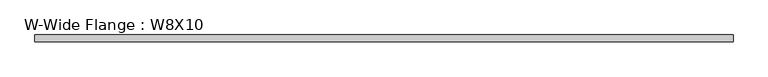
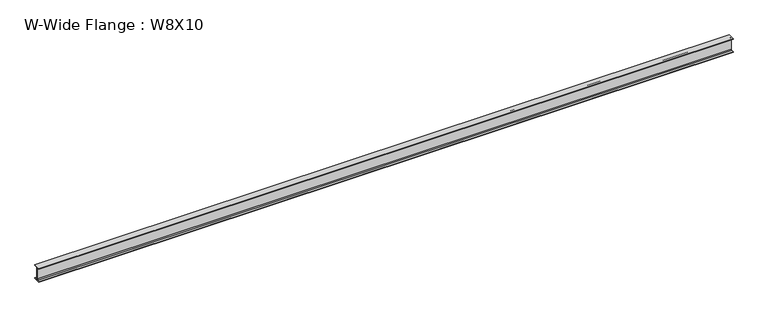
"""IFC4 building model written with IfcOpenShell, lengths in millimetres: beam geometry, W-Wide Flange : W8X10."""

import ifcopenshell
import ifcopenshell.guid

model = None  # the IFC model being written
_history = None  # IfcOwnerHistory: only IFC2X3 demands one
_inside = {}  # id of a spatial element -> (the spatial element, [elements in it])
_under = {}  # id of a project, library or spatial element -> (it, [spatial elements below it])
_declared = {}  # id of a project -> (the project, [libraries it declares])
_typed = {}  # id of a type object -> (the type object, [elements of that type])
_made_of = {}  # id of a material, layer set ... -> (it, [elements and type objects made of it])


def new_model(schema):
    """Start an empty IFC model of exactly this schema.

    Asked for "IFC4X3", IfcOpenShell would pick the latest addendum, in which some entities
    have other attributes; the version numbers below select the first issue.
    IFC2X3 requires an IfcOwnerHistory on every rooted entity: one is made here for all.
    """
    global model, _history
    if schema == "IFC4X3":
        model = ifcopenshell.file(schema_version=(4, 3, 0, 0))
    else:
        model = ifcopenshell.file(schema=schema)
    _inside.clear()
    _under.clear()
    _declared.clear()
    _typed.clear()
    _made_of.clear()
    _history = None
    if model.schema == "IFC2X3":
        org = make("IfcOrganization", Name="unknown")
        user = make(
            "IfcPersonAndOrganization",
            ThePerson=make("IfcPerson", FamilyName="unknown"),
            TheOrganization=org,
        )
        app = make(
            "IfcApplication",
            ApplicationDeveloper=org,
            Version="unknown",
            ApplicationFullName="unknown",
            ApplicationIdentifier="unknown",
        )
        _history = make(
            "IfcOwnerHistory",
            OwningUser=user,
            OwningApplication=app,
            ChangeAction="ADDED",
            CreationDate=0,
        )
    return model


def make(cls, **values):
    """One entity of the class cls with the attributes given. An attribute that is None is left unset."""
    return model.create_entity(
        cls, **{name: value for name, value in values.items() if value is not None}
    )


def rooted(cls, **values):
    """An entity with a GlobalId (a new one), such as an element, a storey or a relation."""
    return make(cls, GlobalId=ifcopenshell.guid.new(), OwnerHistory=_history, **values)


def si_unit(unit_type, name, prefix=None):
    """IfcSIUnit, for example si_unit("LENGTHUNIT", "METRE", prefix="MILLI")."""
    return make("IfcSIUnit", UnitType=unit_type, Prefix=prefix, Name=name)


def assignment(units):
    """IfcUnitAssignment: the units of a project."""
    return None if units is None else make("IfcUnitAssignment", Units=units)


def point(xyz):
    """IfcCartesianPoint."""
    return None if xyz is None else make("IfcCartesianPoint", Coordinates=xyz)


def direction(xyz):
    """IfcDirection."""
    return None if xyz is None else make("IfcDirection", DirectionRatios=xyz)


def frame(location, z_axis=None, x_axis=None):
    """IfcAxis2Placement3D, a coordinate frame: its origin and axes. An axis left out is left unset."""
    return make(
        "IfcAxis2Placement3D",
        Location=point(location),
        Axis=direction(z_axis),
        RefDirection=direction(x_axis),
    )


def frame_2d(location, x_axis=None):
    """IfcAxis2Placement2D, a coordinate frame in the plane: its origin and x axis."""
    return make(
        "IfcAxis2Placement2D", Location=point(location), RefDirection=direction(x_axis)
    )


def origin():
    """The frame at (0, 0, 0) with its axes left unset."""
    return frame((0.0, 0.0, 0.0))


def place(relative_to, where):
    """IfcLocalPlacement: puts the frame where relative to a parent placement (None: the world)."""
    return make(
        "IfcLocalPlacement", PlacementRelTo=relative_to, RelativePlacement=where
    )


def context(
    kind, dimensions, precision=None, world=None, true_north=None, identifier=None
):
    """IfcGeometricRepresentationContext, for example the 3D "Model" context."""
    return make(
        "IfcGeometricRepresentationContext",
        ContextIdentifier=identifier,
        ContextType=kind,
        CoordinateSpaceDimension=dimensions,
        Precision=precision,
        WorldCoordinateSystem=world,
        TrueNorth=true_north,
    )


def project(units=None, contexts=None):
    """IfcProject with its units and contexts."""
    return rooted(
        "IfcProject",
        Name="project",
        RepresentationContexts=contexts,
        UnitsInContext=assignment(units),
    )


def spatial(cls, under=None, at=None, **own):
    """A site, building, storey or space (cls), placed at a placement, below another one or the project."""
    s = rooted(cls, ObjectPlacement=at, **own)
    if under is not None:
        _under.setdefault(under.id(), (under, []))[1].append(s)
    return s


def polyline(points):
    """IfcPolyline through the points."""
    return make("IfcPolyline", Points=[point(p) for p in points])


def circle_curve(where, radius):
    """IfcCircle in the frame where."""
    return make("IfcCircle", Position=where, Radius=radius)


def trimmed(basis, trim1, trim2, sense, master):
    """IfcTrimmedCurve: the piece of a basis curve between two trims."""
    return make(
        "IfcTrimmedCurve",
        BasisCurve=basis,
        Trim1=trim1,
        Trim2=trim2,
        SenseAgreement=sense,
        MasterRepresentation=master,
    )


def segment(curve, same_sense, transition):
    """IfcCompositeCurveSegment."""
    return make(
        "IfcCompositeCurveSegment",
        Transition=transition,
        SameSense=same_sense,
        ParentCurve=curve,
    )


def composite_curve(segments, self_intersect=None):
    """IfcCompositeCurve: segments joined end to end."""
    return make("IfcCompositeCurve", Segments=segments, SelfIntersect=self_intersect)


def outline(outer, holes=None, kind="AREA"):
    """IfcArbitraryClosedProfileDef: a profile drawn as a closed curve; with holes, ...WithVoids."""
    if holes is None:
        return make("IfcArbitraryClosedProfileDef", ProfileType=kind, OuterCurve=outer)
    return make(
        "IfcArbitraryProfileDefWithVoids",
        ProfileType=kind,
        OuterCurve=outer,
        InnerCurves=holes,
    )


def extrude(swept, where, along, depth):
    """IfcExtrudedAreaSolid: the profile swept, set in the frame where, extruded along a direction by depth."""
    return make(
        "IfcExtrudedAreaSolid",
        SweptArea=swept,
        Position=where,
        ExtrudedDirection=direction(along),
        Depth=depth,
    )


def shape(context_of_items, identifier, shape_type, items):
    """IfcShapeRepresentation: the items that make up one representation, for example the "Body"."""
    return make(
        "IfcShapeRepresentation",
        ContextOfItems=context_of_items,
        RepresentationIdentifier=identifier,
        RepresentationType=shape_type,
        Items=items,
    )


def source(mapping_origin, context_of_items, identifier, shape_type, items):
    """IfcRepresentationMap: a shape defined once, which mapped items show again and again."""
    return make(
        "IfcRepresentationMap",
        MappingOrigin=mapping_origin,
        MappedRepresentation=shape(context_of_items, identifier, shape_type, items),
    )


def transform(
    local_origin,
    x_axis=None,
    y_axis=None,
    z_axis=None,
    scale=None,
    scale2=None,
    scale3=None,
    uniform=True,
):
    """IfcCartesianTransformationOperator3D, or its non-uniform kind. x_axis, y_axis, z_axis: its Axis1, 2, 3."""
    if uniform:
        return make(
            "IfcCartesianTransformationOperator3D",
            Axis1=direction(x_axis),
            Axis2=direction(y_axis),
            LocalOrigin=point(local_origin),
            Scale=scale,
            Axis3=direction(z_axis),
        )
    return make(
        "IfcCartesianTransformationOperator3DnonUniform",
        Axis1=direction(x_axis),
        Axis2=direction(y_axis),
        LocalOrigin=point(local_origin),
        Scale=scale,
        Axis3=direction(z_axis),
        Scale2=scale2,
        Scale3=scale3,
    )


def mapped(mapping_source, mapping_target):
    """IfcMappedItem: shows the shape of a source again, moved by a transform."""
    return make(
        "IfcMappedItem", MappingSource=mapping_source, MappingTarget=mapping_target
    )


def made_of(thing, what):
    """Note that an element or type object is made of a material, layer set ...; save() writes the relation."""
    if what is not None:
        _made_of.setdefault(what.id(), (what, []))[1].append(thing)
    return thing


def element(
    cls,
    number,
    at=None,
    inside=None,
    cuts=None,
    type_object=None,
    material=None,
    context=None,
    identifier="Body",
    shape_type=None,
    held_by="IfcProductDefinitionShape",
    body=None,
    shapes=None,
    **own,
):
    """One element of the class cls, such as IfcWall. Its Tag is "e" and its number.

    at: its placement. inside: the storey or other place that contains it. cuts: it is an
    opening in that element (IfcRelVoidsElement). A single representation is given by context,
    identifier, shape_type and body (its items); several are given by shapes. held_by: the class
    of the entity that holds the representations. save() writes the other relations.
    """
    e = rooted(cls, Tag="e%d" % number, ObjectPlacement=at, **own)
    if body is not None:
        shapes = [shape(context, identifier, shape_type, body)]
    if shapes is not None:
        e.Representation = make(held_by, Representations=shapes)
    if inside is not None:
        _inside.setdefault(inside.id(), (inside, []))[1].append(e)
    if cuts is not None:
        rooted(
            "IfcRelVoidsElement", RelatingBuildingElement=cuts, RelatedOpeningElement=e
        )
    if type_object is not None:
        _typed.setdefault(type_object.id(), (type_object, []))[1].append(e)
    return made_of(e, material)


def aggregate(whole, parts):
    """IfcRelAggregates: a whole, such as a stair, and the parts it consists of."""
    return rooted("IfcRelAggregates", RelatingObject=whole, RelatedObjects=parts)


def save(model, path):
    """Write the relations noted so far, then the file.

    IfcRelAggregates (storeys below a building ...), IfcRelContainedInSpatialStructure (elements
    in a storey), IfcRelDefinesByType, IfcRelAssociatesMaterial and IfcRelDeclares: one each for
    every whole, place, type object, material and project.
    """
    for whole, parts in _under.values():
        aggregate(whole, parts)
    for where, things in _inside.values():
        rooted(
            "IfcRelContainedInSpatialStructure",
            RelatedElements=things,
            RelatingStructure=where,
        )
    for kind, things in _typed.values():
        rooted("IfcRelDefinesByType", RelatedObjects=things, RelatingType=kind)
    for what, things in _made_of.values():
        rooted("IfcRelAssociatesMaterial", RelatedObjects=things, RelatingMaterial=what)
    for by, libraries in _declared.values():
        rooted("IfcRelDeclares", RelatingContext=by, RelatedDefinitions=libraries)
    model.write(path)


def w_wide_flange_w8x10_87e04c53(model_context):
    return source(origin(), model_context, "Body", "SweptSolid", [
        extrude(outline(composite_curve([segment(polyline([(50.038, -94.996), (50.038, -100.203), (-50.038, -100.203), (-50.038, -94.996), (-14.4145, -94.996)]), True, "CONTINUOUS"), segment(trimmed(circle_curve(frame_2d((-14.4145, -82.7405)), 12.2555), [point((-14.4145, -94.996))], [point((-2.159, -82.7405))], True, "CARTESIAN"), True, "CONTINUOUS"), segment(polyline([(-2.159, -82.7405), (-2.159, 82.7405)]), True, "CONTINUOUS"), segment(trimmed(circle_curve(frame_2d((-14.4145, 82.7405)), 12.2555), [point((-2.159, 82.7405))], [point((-14.4145, 94.996))], True, "CARTESIAN"), True, "CONTINUOUS"), segment(polyline([(-14.4145, 94.996), (-50.038, 94.996), (-50.038, 100.203), (50.038, 100.203), (50.038, 94.996), (14.4145, 94.996)]), True, "CONTINUOUS"), segment(trimmed(circle_curve(frame_2d((14.4145, 82.7405)), 12.2555), [point((14.4145, 94.996))], [point((2.159, 82.7405))], True, "CARTESIAN"), True, "CONTINUOUS"), segment(polyline([(2.159, 82.7405), (2.159, -82.7405)]), True, "CONTINUOUS"), segment(trimmed(circle_curve(frame_2d((14.4145, -82.7405)), 12.2555), [point((2.159, -82.7405))], [point((14.4145, -94.996))], True, "CARTESIAN"), True, "CONTINUOUS"), segment(polyline([(14.4145, -94.996), (50.038, -94.996)]), True, "CONTINUOUS")], self_intersect=False)), frame((-4974.9523421, 0.0, 0.0), z_axis=(1.0, 0.0, 0.0), x_axis=(0.0, 1.0, 0.0)), (0.0, 0.0, 1.0), 9949.9046843),
    ])


if __name__ == "__main__":
    model = new_model("IFC4")
    model_context = context("Model", 3, world=origin())
    ifc_project = project(units=[si_unit("LENGTHUNIT", "METRE", prefix="MILLI")], contexts=[model_context])
    site = spatial("IfcSite", under=ifc_project)
    building = spatial("IfcBuilding", under=site)
    placement = place(None, origin())
    w_wide_flange_w8x10_shape = w_wide_flange_w8x10_87e04c53(model_context)
    element("IfcBeam", 1, ObjectType="W-Wide Flange : W8X10", at=placement, inside=building, context=model_context, shape_type="MappedRepresentation", body=[
        mapped(w_wide_flange_w8x10_shape, transform((0.0, 0.0, 0.0), x_axis=(1.0, 0.0, 0.0), y_axis=(0.0, 1.0, 0.0), z_axis=(0.0, 0.0, 1.0))),
    ])
    save(model, "model.ifc")

# Revit data of these elements
# Type "W-Wide Flange : W8X10"
#   Assembly Code = "B10"
#   W = 10
#   Length [instance default] = 5' - 0"
#   bf = 0' - 3.94"
#   d = 0' - 7.89"
#   k = 0' - 0 11/16"
#   k2 = 0' - 0.4825"
#   tf = 0' - 0.205"
#   tw = 0' - 0.17"
#   A = 0.0205556 SF
#   Structural Material [instance default] = Steel ASTM A992
# Element 1 (IfcBeam, "W-Wide Flange : W8X10")
#   Structural Material = none
# Materials
#   "Steel ASTM A992": class "Metal", colour RGB 189 187 185, transparency 0, Description = "Structural steel 50ksi", Cost = 0
